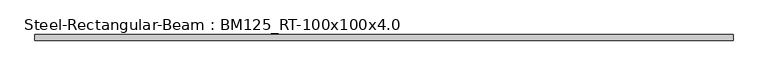
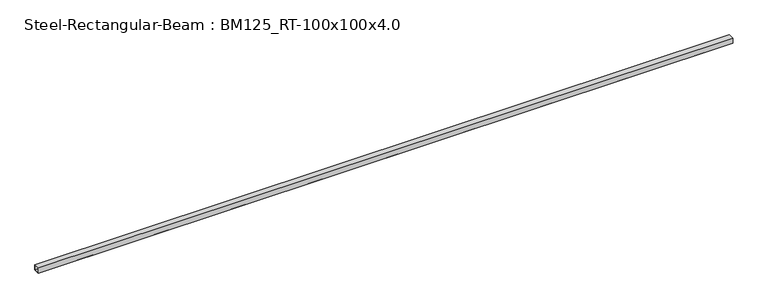
"""IFC4 building model written with IfcOpenShell, lengths in millimetres: beam geometry, Steel-Rectangular-Beam : BM125_RT-100x100x4.0."""

import ifcopenshell
import ifcopenshell.guid

model = None  # the IFC model being written
_history = None  # IfcOwnerHistory: only IFC2X3 demands one
_inside = {}  # id of a spatial element -> (the spatial element, [elements in it])
_under = {}  # id of a project, library or spatial element -> (it, [spatial elements below it])
_declared = {}  # id of a project -> (the project, [libraries it declares])
_typed = {}  # id of a type object -> (the type object, [elements of that type])
_made_of = {}  # id of a material, layer set ... -> (it, [elements and type objects made of it])


def new_model(schema):
    """Start an empty IFC model of exactly this schema.

    Asked for "IFC4X3", IfcOpenShell would pick the latest addendum, in which some entities
    have other attributes; the version numbers below select the first issue.
    IFC2X3 requires an IfcOwnerHistory on every rooted entity: one is made here for all.
    """
    global model, _history
    if schema == "IFC4X3":
        model = ifcopenshell.file(schema_version=(4, 3, 0, 0))
    else:
        model = ifcopenshell.file(schema=schema)
    _inside.clear()
    _under.clear()
    _declared.clear()
    _typed.clear()
    _made_of.clear()
    _history = None
    if model.schema == "IFC2X3":
        org = make("IfcOrganization", Name="unknown")
        user = make(
            "IfcPersonAndOrganization",
            ThePerson=make("IfcPerson", FamilyName="unknown"),
            TheOrganization=org,
        )
        app = make(
            "IfcApplication",
            ApplicationDeveloper=org,
            Version="unknown",
            ApplicationFullName="unknown",
            ApplicationIdentifier="unknown",
        )
        _history = make(
            "IfcOwnerHistory",
            OwningUser=user,
            OwningApplication=app,
            ChangeAction="ADDED",
            CreationDate=0,
        )
    return model


def make(cls, **values):
    """One entity of the class cls with the attributes given. An attribute that is None is left unset."""
    return model.create_entity(
        cls, **{name: value for name, value in values.items() if value is not None}
    )


def rooted(cls, **values):
    """An entity with a GlobalId (a new one), such as an element, a storey or a relation."""
    return make(cls, GlobalId=ifcopenshell.guid.new(), OwnerHistory=_history, **values)


def si_unit(unit_type, name, prefix=None):
    """IfcSIUnit, for example si_unit("LENGTHUNIT", "METRE", prefix="MILLI")."""
    return make("IfcSIUnit", UnitType=unit_type, Prefix=prefix, Name=name)


def assignment(units):
    """IfcUnitAssignment: the units of a project."""
    return None if units is None else make("IfcUnitAssignment", Units=units)


def point(xyz):
    """IfcCartesianPoint."""
    return None if xyz is None else make("IfcCartesianPoint", Coordinates=xyz)


def direction(xyz):
    """IfcDirection."""
    return None if xyz is None else make("IfcDirection", DirectionRatios=xyz)


def frame(location, z_axis=None, x_axis=None):
    """IfcAxis2Placement3D, a coordinate frame: its origin and axes. An axis left out is left unset."""
    return make(
        "IfcAxis2Placement3D",
        Location=point(location),
        Axis=direction(z_axis),
        RefDirection=direction(x_axis),
    )


def origin():
    """The frame at (0, 0, 0) with its axes left unset."""
    return frame((0.0, 0.0, 0.0))


def place(relative_to, where):
    """IfcLocalPlacement: puts the frame where relative to a parent placement (None: the world)."""
    return make(
        "IfcLocalPlacement", PlacementRelTo=relative_to, RelativePlacement=where
    )


def context(
    kind, dimensions, precision=None, world=None, true_north=None, identifier=None
):
    """IfcGeometricRepresentationContext, for example the 3D "Model" context."""
    return make(
        "IfcGeometricRepresentationContext",
        ContextIdentifier=identifier,
        ContextType=kind,
        CoordinateSpaceDimension=dimensions,
        Precision=precision,
        WorldCoordinateSystem=world,
        TrueNorth=true_north,
    )


def project(units=None, contexts=None):
    """IfcProject with its units and contexts."""
    return rooted(
        "IfcProject",
        Name="project",
        RepresentationContexts=contexts,
        UnitsInContext=assignment(units),
    )


def spatial(cls, under=None, at=None, **own):
    """A site, building, storey or space (cls), placed at a placement, below another one or the project."""
    s = rooted(cls, ObjectPlacement=at, **own)
    if under is not None:
        _under.setdefault(under.id(), (under, []))[1].append(s)
    return s


def polyline(points):
    """IfcPolyline through the points."""
    return make("IfcPolyline", Points=[point(p) for p in points])


def outline(outer, holes=None, kind="AREA"):
    """IfcArbitraryClosedProfileDef: a profile drawn as a closed curve; with holes, ...WithVoids."""
    if holes is None:
        return make("IfcArbitraryClosedProfileDef", ProfileType=kind, OuterCurve=outer)
    return make(
        "IfcArbitraryProfileDefWithVoids",
        ProfileType=kind,
        OuterCurve=outer,
        InnerCurves=holes,
    )


def extrude(swept, where, along, depth):
    """IfcExtrudedAreaSolid: the profile swept, set in the frame where, extruded along a direction by depth."""
    return make(
        "IfcExtrudedAreaSolid",
        SweptArea=swept,
        Position=where,
        ExtrudedDirection=direction(along),
        Depth=depth,
    )


def shape(context_of_items, identifier, shape_type, items):
    """IfcShapeRepresentation: the items that make up one representation, for example the "Body"."""
    return make(
        "IfcShapeRepresentation",
        ContextOfItems=context_of_items,
        RepresentationIdentifier=identifier,
        RepresentationType=shape_type,
        Items=items,
    )


def source(mapping_origin, context_of_items, identifier, shape_type, items):
    """IfcRepresentationMap: a shape defined once, which mapped items show again and again."""
    return make(
        "IfcRepresentationMap",
        MappingOrigin=mapping_origin,
        MappedRepresentation=shape(context_of_items, identifier, shape_type, items),
    )


def transform(
    local_origin,
    x_axis=None,
    y_axis=None,
    z_axis=None,
    scale=None,
    scale2=None,
    scale3=None,
    uniform=True,
):
    """IfcCartesianTransformationOperator3D, or its non-uniform kind. x_axis, y_axis, z_axis: its Axis1, 2, 3."""
    if uniform:
        return make(
            "IfcCartesianTransformationOperator3D",
            Axis1=direction(x_axis),
            Axis2=direction(y_axis),
            LocalOrigin=point(local_origin),
            Scale=scale,
            Axis3=direction(z_axis),
        )
    return make(
        "IfcCartesianTransformationOperator3DnonUniform",
        Axis1=direction(x_axis),
        Axis2=direction(y_axis),
        LocalOrigin=point(local_origin),
        Scale=scale,
        Axis3=direction(z_axis),
        Scale2=scale2,
        Scale3=scale3,
    )


def mapped(mapping_source, mapping_target):
    """IfcMappedItem: shows the shape of a source again, moved by a transform."""
    return make(
        "IfcMappedItem", MappingSource=mapping_source, MappingTarget=mapping_target
    )


def made_of(thing, what):
    """Note that an element or type object is made of a material, layer set ...; save() writes the relation."""
    if what is not None:
        _made_of.setdefault(what.id(), (what, []))[1].append(thing)
    return thing


def element(
    cls,
    number,
    at=None,
    inside=None,
    cuts=None,
    type_object=None,
    material=None,
    context=None,
    identifier="Body",
    shape_type=None,
    held_by="IfcProductDefinitionShape",
    body=None,
    shapes=None,
    **own,
):
    """One element of the class cls, such as IfcWall. Its Tag is "e" and its number.

    at: its placement. inside: the storey or other place that contains it. cuts: it is an
    opening in that element (IfcRelVoidsElement). A single representation is given by context,
    identifier, shape_type and body (its items); several are given by shapes. held_by: the class
    of the entity that holds the representations. save() writes the other relations.
    """
    e = rooted(cls, Tag="e%d" % number, ObjectPlacement=at, **own)
    if body is not None:
        shapes = [shape(context, identifier, shape_type, body)]
    if shapes is not None:
        e.Representation = make(held_by, Representations=shapes)
    if inside is not None:
        _inside.setdefault(inside.id(), (inside, []))[1].append(e)
    if cuts is not None:
        rooted(
            "IfcRelVoidsElement", RelatingBuildingElement=cuts, RelatedOpeningElement=e
        )
    if type_object is not None:
        _typed.setdefault(type_object.id(), (type_object, []))[1].append(e)
    return made_of(e, material)


def aggregate(whole, parts):
    """IfcRelAggregates: a whole, such as a stair, and the parts it consists of."""
    return rooted("IfcRelAggregates", RelatingObject=whole, RelatedObjects=parts)


def save(model, path):
    """Write the relations noted so far, then the file.

    IfcRelAggregates (storeys below a building ...), IfcRelContainedInSpatialStructure (elements
    in a storey), IfcRelDefinesByType, IfcRelAssociatesMaterial and IfcRelDeclares: one each for
    every whole, place, type object, material and project.
    """
    for whole, parts in _under.values():
        aggregate(whole, parts)
    for where, things in _inside.values():
        rooted(
            "IfcRelContainedInSpatialStructure",
            RelatedElements=things,
            RelatingStructure=where,
        )
    for kind, things in _typed.values():
        rooted("IfcRelDefinesByType", RelatedObjects=things, RelatingType=kind)
    for what, things in _made_of.values():
        rooted("IfcRelAssociatesMaterial", RelatedObjects=things, RelatingMaterial=what)
    for by, libraries in _declared.values():
        rooted("IfcRelDeclares", RelatingContext=by, RelatedDefinitions=libraries)
    model.write(path)


def steel_rectangular_beam_bm125_rt_100x100x4_0_88b81966(model_context):
    return source(origin(), model_context, "Body", "SweptSolid", [
        extrude(outline(polyline([(-50.0, 50.0), (50.0, 50.0), (50.0, -50.0), (-50.0, -50.0), (-50.0, 50.0)]), holes=[polyline([(46.0, -46.0), (46.0, 46.0), (-46.0, 46.0), (-46.0, -46.0), (46.0, -46.0)])]), frame((-6200.0, 0.0, 0.0), z_axis=(1.0, 0.0, 0.0), x_axis=(0.0, 1.0, 0.0)), (0.0, 0.0, 1.0), 12400.0),
        extrude(outline(polyline([(-50.0, 50.0), (50.0, 50.0), (50.0, -50.0), (-50.0, -50.0), (-50.0, 50.0)]), holes=[polyline([(46.0, -46.0), (46.0, 46.0), (-46.0, 46.0), (-46.0, -46.0), (46.0, -46.0)])]), frame((-6200.0, 0.0, 0.0), z_axis=(1.0, 0.0, 0.0), x_axis=(0.0, 1.0, 0.0)), (0.0, 0.0, 1.0), 12400.0),
        extrude(outline(polyline([(-50.0, 50.0), (50.0, 50.0), (50.0, -50.0), (-50.0, -50.0), (-50.0, 50.0)]), holes=[polyline([(46.0, -46.0), (46.0, 46.0), (-46.0, 46.0), (-46.0, -46.0), (46.0, -46.0)])]), frame((-6200.0, 0.0, 0.0), z_axis=(1.0, 0.0, 0.0), x_axis=(0.0, 1.0, 0.0)), (0.0, 0.0, 1.0), 12400.0),
        extrude(outline(polyline([(-50.0, 50.0), (50.0, 50.0), (50.0, -50.0), (-50.0, -50.0), (-50.0, 50.0)]), holes=[polyline([(46.0, -46.0), (46.0, 46.0), (-46.0, 46.0), (-46.0, -46.0), (46.0, -46.0)])]), frame((-6200.0, 0.0, 0.0), z_axis=(1.0, 0.0, 0.0), x_axis=(0.0, 1.0, 0.0)), (0.0, 0.0, 1.0), 12400.0),
    ])


if __name__ == "__main__":
    model = new_model("IFC4")
    model_context = context("Model", 3, world=origin())
    ifc_project = project(units=[si_unit("LENGTHUNIT", "METRE", prefix="MILLI")], contexts=[model_context])
    site = spatial("IfcSite", under=ifc_project)
    building = spatial("IfcBuilding", under=site)
    placement = place(None, origin())
    steel_rectangular_beam_bm125_rt_100x100x4_0_shape = steel_rectangular_beam_bm125_rt_100x100x4_0_88b81966(model_context)
    element("IfcBeam", 1, ObjectType="Steel-Rectangular-Beam : BM125_RT-100x100x4.0", at=placement, inside=building, context=model_context, shape_type="MappedRepresentation", body=[
        mapped(steel_rectangular_beam_bm125_rt_100x100x4_0_shape, transform((0.0, 0.0, 0.0), x_axis=(1.0, 0.0, 0.0), y_axis=(0.0, 1.0, 0.0), z_axis=(0.0, 0.0, 1.0))),
    ])
    save(model, "model.ifc")

# Revit data of these elements
# Type "Steel-Rectangular-Beam : BM125_RT-100x100x4.0"
#   t = 4 mm
#   Mass per Unit Length = 11.70 kg/m
#   Surface Area = 0.386 m²/m
#   Sectional Area = 14.95 cm²
#   Length [instance default] = 3000 mm
#   H = 100 mm
#   B = 100 mm
#   hec_material4 [instance default] = none
#   hec_material3 [instance default] = none
#   hec_material2 [instance default] = none
#   hec_material1 [instance default] = none
#   Structural Material [instance default] = none
# Element 1 (IfcBeam, "Steel-Rectangular-Beam : BM125_RT-100x100x4.0")
#   hec_material2 = S01AA010-00001_Main Steel Structure Fabrication Work_Shelter/Building_Steel Painting/Coating_for Non-Fireproofed Steel Surface, Surface Preparation, Primer, Second & Final Coat
#   hec_material1 = S03AA007-00001_Main Steel Structure Erection Work_Girth & Purlin
#   Structural Material = S01AA007-00001_Main Steel Structure Fabrication Work_Shelter/Building_Girth & Purlin
#   Materials on its faces: "S01AA010-00001_Main Steel Structure Fabrication Work_Shelter/Building_Steel Painting/Coating_for Non-Fireproofed Steel Surface, Surface Preparation, Primer, Second & Final Coat"
# Materials
#   "S01AA010-00001_Main Steel Structure Fabrication Work_Shelter/Building_Steel Painting/Coating_for Non-Fireproofed Steel Surface, Surface Preparation, Primer, Second & Final Coat": class "Metal", colour RGB 120 120 120, transparency 0, Description = "Paint finished steel", W00) Work Master Code = "S01AA010-00001", W01) Work Master_Lv1 = "Main Steel Structure Fabrication Work", W02) Work Master_Lv2 = "Shelter/Building", W03) Work Master_Spec.1 = "Steel Painting/Coating", W04) Work Master_Spec.2 = "for Non-Fireproofed Steel Surface, Surface Preparation, Primer, Second & Final Coat", Cost = 0
#   "S03AA007-00001_Main Steel Structure Erection Work_Girth & Purlin": class "Metal", colour RGB 120 120 120, transparency 0, Comments = "(30KG/M>Weight)", Description = "Structural steel 50ksi", W00) Work Master Code = "S03AA007-00001", W01) Work Master_Lv1 = "Main Steel Structure Erection Work", W02) Work Master_Lv2 = "Shelter/Building", W03) Work Master_Spec.1 = "Girth & Purlin", Cost = 0
#   "S01AA007-00001_Main Steel Structure Fabrication Work_Shelter/Building_Girth & Purlin": class "Metal", colour RGB 120 120 120, transparency 0, Comments = "(30KG/M>Weight)", Description = "Structural steel 50ksi", W00) Work Master Code = "S01AA007-00001", W01) Work Master_Lv1 = "Main Steel Structure Fabrication Work", W02) Work Master_Lv2 = "Shelter/Building", W03) Work Master_Spec.1 = "Girth & Purlin", Cost = 0
